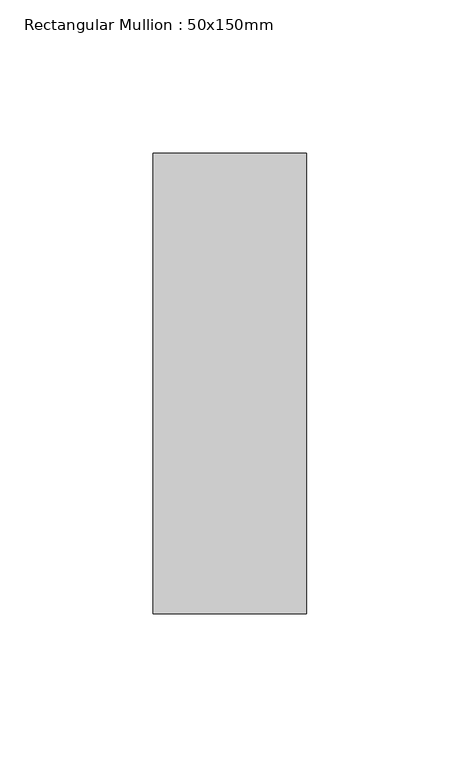
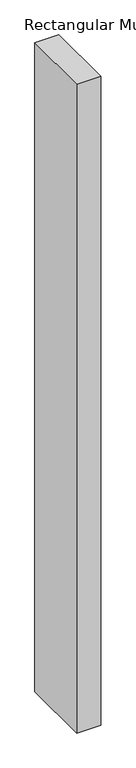
"""IFC4 building model written with IfcOpenShell, lengths in millimetres: member geometry, Rectangular Mullion : 50x150mm."""

from ifc_helpers import new_model, si_unit, frame, origin, place, context, project, spatial, polyline, outline, extrude, source, transform, mapped, element, save


def rectangular_mullion_50x150mm_2a0b7483(model_context):
    return source(origin(), model_context, "Body", "SweptSolid", [
        extrude(outline(polyline([(0.0, 75.0), (0.0, -75.0), (-50.0, -75.0), (-50.0, 75.0), (0.0, 75.0)])), frame((0.0, 0.0, -1425.0000002), z_axis=(0.0, 0.0, 1.0), x_axis=(1.0, 0.0, 0.0)), (0.0, 0.0, 1.0), 1425.0000002),
    ])


if __name__ == "__main__":
    model = new_model("IFC4")
    model_context = context("Model", 3, world=origin())
    ifc_project = project(units=[si_unit("LENGTHUNIT", "METRE", prefix="MILLI")], contexts=[model_context])
    site = spatial("IfcSite", under=ifc_project)
    building = spatial("IfcBuilding", under=site)
    placement = place(None, origin())
    rectangular_mullion_50x150mm_shape = rectangular_mullion_50x150mm_2a0b7483(model_context)
    element("IfcMember", 1, ObjectType="Rectangular Mullion : 50x150mm", at=placement, inside=building, context=model_context, shape_type="MappedRepresentation", body=[
        mapped(rectangular_mullion_50x150mm_shape, transform((0.0, 0.0, 0.0), x_axis=(1.0, 0.0, 0.0), y_axis=(0.0, 1.0, 0.0), z_axis=(0.0, 0.0, 1.0))),
    ])
    save(model, "model.ifc")

# Revit data of these elements
# Type "Rectangular Mullion : 50x150mm"
#   Keynote = "H11"
#   built-in parameter 1007304 = 0.492126 (stored number, unit not read)
#   built-in parameter 1007301 = 0.082021 (stored number, unit not read)
#   built-in parameter 1007300 = 0.082021 (stored number, unit not read)
# Element 1 (IfcMember, "Rectangular Mullion : 50x150mm")
#   Materials on its faces: "Aluminium"
# Materials
#   "Aluminium": class "Metal", colour RGB 247 247 247, transparency 0, Description = "Aluminium 6061", Cost = 0
